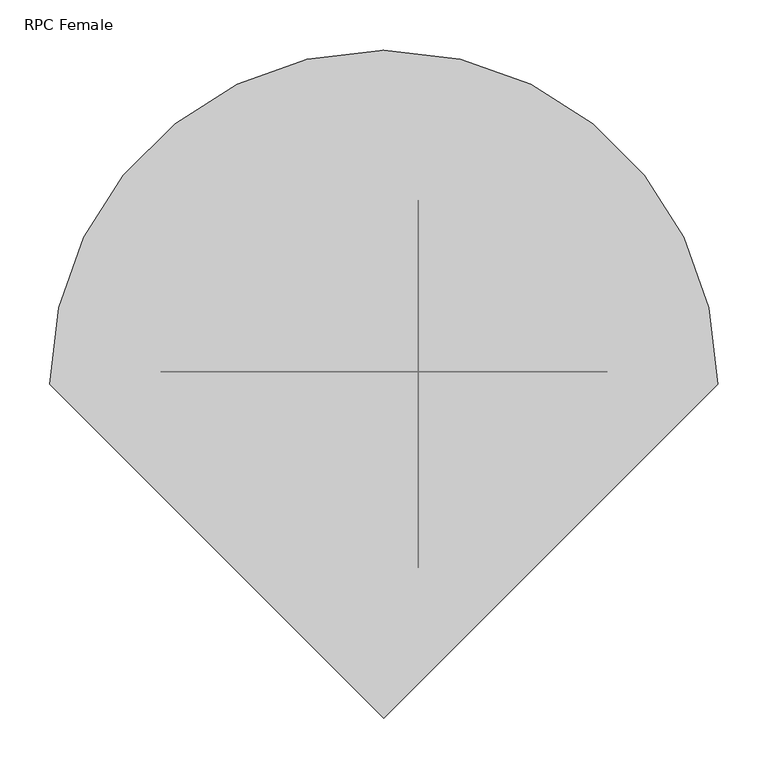
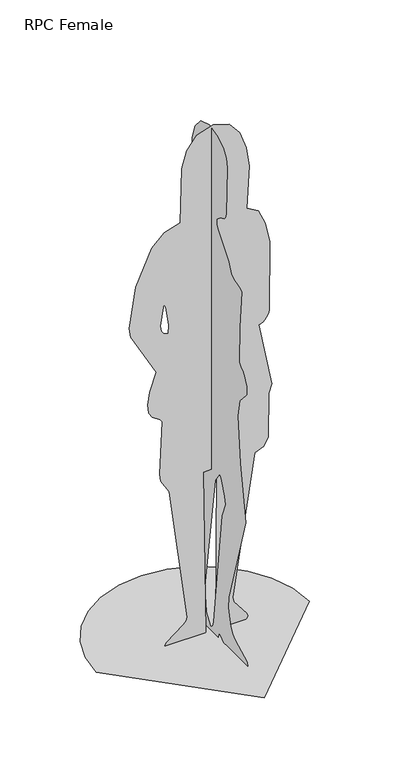
"""IFC4 building model written with IfcOpenShell, lengths in millimetres: proxy geometry, RPC Female : Florence."""

import ifcopenshell
import ifcopenshell.guid

model = None  # the IFC model being written
_history = None  # IfcOwnerHistory: only IFC2X3 demands one
_inside = {}  # id of a spatial element -> (the spatial element, [elements in it])
_under = {}  # id of a project, library or spatial element -> (it, [spatial elements below it])
_declared = {}  # id of a project -> (the project, [libraries it declares])
_typed = {}  # id of a type object -> (the type object, [elements of that type])
_made_of = {}  # id of a material, layer set ... -> (it, [elements and type objects made of it])


def new_model(schema):
    """Start an empty IFC model of exactly this schema.

    Asked for "IFC4X3", IfcOpenShell would pick the latest addendum, in which some entities
    have other attributes; the version numbers below select the first issue.
    IFC2X3 requires an IfcOwnerHistory on every rooted entity: one is made here for all.
    """
    global model, _history
    if schema == "IFC4X3":
        model = ifcopenshell.file(schema_version=(4, 3, 0, 0))
    else:
        model = ifcopenshell.file(schema=schema)
    _inside.clear()
    _under.clear()
    _declared.clear()
    _typed.clear()
    _made_of.clear()
    _history = None
    if model.schema == "IFC2X3":
        org = make("IfcOrganization", Name="unknown")
        user = make(
            "IfcPersonAndOrganization",
            ThePerson=make("IfcPerson", FamilyName="unknown"),
            TheOrganization=org,
        )
        app = make(
            "IfcApplication",
            ApplicationDeveloper=org,
            Version="unknown",
            ApplicationFullName="unknown",
            ApplicationIdentifier="unknown",
        )
        _history = make(
            "IfcOwnerHistory",
            OwningUser=user,
            OwningApplication=app,
            ChangeAction="ADDED",
            CreationDate=0,
        )
    return model


def make(cls, **values):
    """One entity of the class cls with the attributes given. An attribute that is None is left unset."""
    return model.create_entity(
        cls, **{name: value for name, value in values.items() if value is not None}
    )


def rooted(cls, **values):
    """An entity with a GlobalId (a new one), such as an element, a storey or a relation."""
    return make(cls, GlobalId=ifcopenshell.guid.new(), OwnerHistory=_history, **values)


def si_unit(unit_type, name, prefix=None):
    """IfcSIUnit, for example si_unit("LENGTHUNIT", "METRE", prefix="MILLI")."""
    return make("IfcSIUnit", UnitType=unit_type, Prefix=prefix, Name=name)


def assignment(units):
    """IfcUnitAssignment: the units of a project."""
    return None if units is None else make("IfcUnitAssignment", Units=units)


def point(xyz):
    """IfcCartesianPoint."""
    return None if xyz is None else make("IfcCartesianPoint", Coordinates=xyz)


def direction(xyz):
    """IfcDirection."""
    return None if xyz is None else make("IfcDirection", DirectionRatios=xyz)


def frame(location, z_axis=None, x_axis=None):
    """IfcAxis2Placement3D, a coordinate frame: its origin and axes. An axis left out is left unset."""
    return make(
        "IfcAxis2Placement3D",
        Location=point(location),
        Axis=direction(z_axis),
        RefDirection=direction(x_axis),
    )


def origin():
    """The frame at (0, 0, 0) with its axes left unset."""
    return frame((0.0, 0.0, 0.0))


def place(relative_to, where):
    """IfcLocalPlacement: puts the frame where relative to a parent placement (None: the world)."""
    return make(
        "IfcLocalPlacement", PlacementRelTo=relative_to, RelativePlacement=where
    )


def context(
    kind, dimensions, precision=None, world=None, true_north=None, identifier=None
):
    """IfcGeometricRepresentationContext, for example the 3D "Model" context."""
    return make(
        "IfcGeometricRepresentationContext",
        ContextIdentifier=identifier,
        ContextType=kind,
        CoordinateSpaceDimension=dimensions,
        Precision=precision,
        WorldCoordinateSystem=world,
        TrueNorth=true_north,
    )


def project(units=None, contexts=None):
    """IfcProject with its units and contexts."""
    return rooted(
        "IfcProject",
        Name="project",
        RepresentationContexts=contexts,
        UnitsInContext=assignment(units),
    )


def spatial(cls, under=None, at=None, **own):
    """A site, building, storey or space (cls), placed at a placement, below another one or the project."""
    s = rooted(cls, ObjectPlacement=at, **own)
    if under is not None:
        _under.setdefault(under.id(), (under, []))[1].append(s)
    return s


def point_list(points):
    """IfcCartesianPointList2D or 3D."""
    cls = (
        "IfcCartesianPointList2D" if len(points[0]) == 2 else "IfcCartesianPointList3D"
    )
    return make(cls, CoordList=points)


def triangles(points, corners, closed=None, point_numbers=None):
    """IfcTriangulatedFaceSet: each triangle names its three corners, points numbered from 1."""
    return make(
        "IfcTriangulatedFaceSet",
        Coordinates=point_list(points),
        Closed=closed,
        CoordIndex=corners,
        PnIndex=point_numbers,
    )


def shape(context_of_items, identifier, shape_type, items):
    """IfcShapeRepresentation: the items that make up one representation, for example the "Body"."""
    return make(
        "IfcShapeRepresentation",
        ContextOfItems=context_of_items,
        RepresentationIdentifier=identifier,
        RepresentationType=shape_type,
        Items=items,
    )


def source(mapping_origin, context_of_items, identifier, shape_type, items):
    """IfcRepresentationMap: a shape defined once, which mapped items show again and again."""
    return make(
        "IfcRepresentationMap",
        MappingOrigin=mapping_origin,
        MappedRepresentation=shape(context_of_items, identifier, shape_type, items),
    )


def transform(
    local_origin,
    x_axis=None,
    y_axis=None,
    z_axis=None,
    scale=None,
    scale2=None,
    scale3=None,
    uniform=True,
):
    """IfcCartesianTransformationOperator3D, or its non-uniform kind. x_axis, y_axis, z_axis: its Axis1, 2, 3."""
    if uniform:
        return make(
            "IfcCartesianTransformationOperator3D",
            Axis1=direction(x_axis),
            Axis2=direction(y_axis),
            LocalOrigin=point(local_origin),
            Scale=scale,
            Axis3=direction(z_axis),
        )
    return make(
        "IfcCartesianTransformationOperator3DnonUniform",
        Axis1=direction(x_axis),
        Axis2=direction(y_axis),
        LocalOrigin=point(local_origin),
        Scale=scale,
        Axis3=direction(z_axis),
        Scale2=scale2,
        Scale3=scale3,
    )


def mapped(mapping_source, mapping_target):
    """IfcMappedItem: shows the shape of a source again, moved by a transform."""
    return make(
        "IfcMappedItem", MappingSource=mapping_source, MappingTarget=mapping_target
    )


def made_of(thing, what):
    """Note that an element or type object is made of a material, layer set ...; save() writes the relation."""
    if what is not None:
        _made_of.setdefault(what.id(), (what, []))[1].append(thing)
    return thing


def element(
    cls,
    number,
    at=None,
    inside=None,
    cuts=None,
    type_object=None,
    material=None,
    context=None,
    identifier="Body",
    shape_type=None,
    held_by="IfcProductDefinitionShape",
    body=None,
    shapes=None,
    **own,
):
    """One element of the class cls, such as IfcWall. Its Tag is "e" and its number.

    at: its placement. inside: the storey or other place that contains it. cuts: it is an
    opening in that element (IfcRelVoidsElement). A single representation is given by context,
    identifier, shape_type and body (its items); several are given by shapes. held_by: the class
    of the entity that holds the representations. save() writes the other relations.
    """
    e = rooted(cls, Tag="e%d" % number, ObjectPlacement=at, **own)
    if body is not None:
        shapes = [shape(context, identifier, shape_type, body)]
    if shapes is not None:
        e.Representation = make(held_by, Representations=shapes)
    if inside is not None:
        _inside.setdefault(inside.id(), (inside, []))[1].append(e)
    if cuts is not None:
        rooted(
            "IfcRelVoidsElement", RelatingBuildingElement=cuts, RelatedOpeningElement=e
        )
    if type_object is not None:
        _typed.setdefault(type_object.id(), (type_object, []))[1].append(e)
    return made_of(e, material)


def aggregate(whole, parts):
    """IfcRelAggregates: a whole, such as a stair, and the parts it consists of."""
    return rooted("IfcRelAggregates", RelatingObject=whole, RelatedObjects=parts)


def save(model, path):
    """Write the relations noted so far, then the file.

    IfcRelAggregates (storeys below a building ...), IfcRelContainedInSpatialStructure (elements
    in a storey), IfcRelDefinesByType, IfcRelAssociatesMaterial and IfcRelDeclares: one each for
    every whole, place, type object, material and project.
    """
    for whole, parts in _under.values():
        aggregate(whole, parts)
    for where, things in _inside.values():
        rooted(
            "IfcRelContainedInSpatialStructure",
            RelatedElements=things,
            RelatingStructure=where,
        )
    for kind, things in _typed.values():
        rooted("IfcRelDefinesByType", RelatedObjects=things, RelatingType=kind)
    for what, things in _made_of.values():
        rooted("IfcRelAssociatesMaterial", RelatedObjects=things, RelatingMaterial=what)
    for by, libraries in _declared.values():
        rooted("IfcRelDeclares", RelatingContext=by, RelatedDefinitions=libraries)
    model.write(path)


def rpc_female_692637f3(model_context):
    return source(origin(), model_context, "Body", "Tessellation", [
        triangles([(334.1038436, 0.0002006, 4.67e-05), (325.2712069, 76.554684, 4.67e-05), (300.1160563, 146.8577329, 4.67e-05), (260.6525312, 208.8950799, 4.67e-05), (208.8950436, 260.6526402, 4.67e-05), (146.8576239, 300.1161108, 4.67e-05), (76.5545841, 325.2713159, 4.67e-05), (0.0001119, 334.1039526, 4.67e-05), (-76.5543661, 325.2713159, 4.67e-05), (-146.8574241, 300.1161471, 4.67e-05), (-208.8947893, 260.6526402, 4.67e-05), (-260.6523677, 208.8951526, 4.67e-05), (-300.1157837, 146.8577238, 4.67e-05), (-325.2709888, 76.5546749, 4.67e-05), (-334.1036256, 0.0002063, 4.67e-05), (0.0001354, -334.1035166, 4.67e-05), (34.5735982, -6.9369908, 510.5862036), (34.5736005, 50.0894208, 122.5869578), (34.5736005, 40.8608144, 46.3929486), (34.5735982, 17.1569787, 11.3406073), (34.5735982, 7.4077424, 20.0668393), (34.5735982, 1.2816647, 37.4286861), (34.5735982, -2.1837537, 60.406083), (34.573596, -46.4921976, 417.5145226), (34.573596, -63.110333, 464.5403223), (34.573596, -60.1161389, 490.2851171), (34.573596, -39.0453865, 536.4626401), (34.573596, -31.9759211, 546.3433597), (34.5736051, 133.6635619, 4.67e-05), (34.5736051, 131.2497012, 427.6552917), (34.5736028, 105.4428553, 516.402818), (34.5736051, 133.6330768, 904.8776161), (34.5736051, 118.5363239, 971.9484495), (34.5736051, 119.0610557, 980.9675211), (34.5736051, 126.7253499, 988.4865389), (34.5736073, 167.3251791, 1010.3459604), (34.5736073, 178.3172225, 1020.1671633), (34.5736073, 183.8335464, 1032.6394398), (34.5736073, 170.1064229, 1269.4988194), (34.5736073, 153.1875791, 1316.4971134), (34.5736051, 126.3412163, 1357.63312), (34.5736051, 116.7179574, 1573.3395756), (34.5736028, 100.9948892, 1620.5182365), (34.5736028, 71.8814228, 1654.7582977), (34.5736005, 25.3458139, 1670.9407402), (34.573596, -21.8028775, 1659.2649994), (34.573596, -51.3715418, 1640.0022217), (34.5735937, -67.2787558, 1615.437006), (34.5735937, -73.4430507, 1587.8543873), (34.5735937, -67.1164838, 1429.4550442), (34.573596, -62.6125163, 1414.6470818), (34.573596, -56.0058929, 1408.6359661), (34.573596, -33.6371819, 1398.6160835), (34.5735982, -16.4512737, 1382.4130028), (34.5735982, -16.5742143, 1366.5170254), (34.573596, -23.8041702, 1350.9894848), (34.5735937, -80.3271009, 1279.6723263), (34.5735937, -93.6682833, 1248.0555061), (34.5735937, -101.8993307, 1241.9481754), (34.5735914, -113.2375739, 1237.3922035), (34.5735914, -125.7355211, 1233.7834122), (34.5735914, -137.445871, 1230.5184952), (34.5735914, -146.4210681, 1226.9929836), (34.5735914, -150.7137475, 1222.6031353), (34.5735914, -148.5625071, 1190.0747429), (34.5735914, -140.3131288, 1099.0845119), (34.5735914, -138.7464003, 982.8324509), (34.5735914, -146.619339, 972.1617359), (34.5735892, -156.6982296, 965.1524254), (34.5735892, -165.5360078, 953.6295095), (34.5735892, -177.5233393, 924.4368147), (34.5735892, -179.6904672, 910.463249), (34.5735892, -178.6515408, 899.3693041), (34.5735892, -173.9153837, 893.0032682), (34.5735914, -141.1932077, 856.8173229), (34.5735914, -128.9730324, 798.8474602), (34.5735914, -142.8069082, 650.4621861), (34.5735892, -172.1239596, 470.1701385), (34.5735937, -80.165383, 167.8524907), (34.5735937, -77.6113328, 131.7844796), (34.5735937, -91.6647991, 75.8743931), (34.5735937, -102.4531668, 58.8461219), (34.5735914, -116.401843, 46.2735109), (34.5735892, -182.1041825, 14.070202), (34.5735892, -183.8332739, 4.67e-05), (34.573596, -53.8341595, 4.67e-05), (34.573596, -35.7947333, 12.7326758), (34.573596, -29.2463276, 15.4350465), (34.573596, -27.5084158, 14.8404334), (34.573596, -26.3930815, 13.6010264), (34.573596, -23.0174154, 4.67e-05), (-109.094313, 12.6252593, 1123.2807821), (-99.0692164, 12.6252548, 1062.4456146), (-101.4218071, 12.6252536, 1032.213085), (-115.6875607, 12.6252536, 1036.9381599), (-123.3610839, 12.6252559, 1049.3745375), (-125.9345188, 12.6252559, 1066.9140919), (-115.0698113, 12.6252593, 1135.9380037), (142.5673516, 12.6251787, 0.0), (147.4016405, 12.6251787, 9.7557227), (144.3531438, 12.6251798, 20.3925416), (104.8323548, 12.6251855, 72.3575519), (100.9956885, 12.6251855, 87.8546938), (169.3636811, 12.6252093, 543.0591125), (197.666532, 12.6252093, 555.605367), (211.7994085, 12.6252093, 579.9655443), (214.3379708, 12.6252173, 724.0128565), (223.4012803, 12.6252196, 753.7932335), (181.7748058, 12.6252343, 962.6080313), (189.3709628, 12.6252332, 963.9546787), (195.9600047, 12.6252332, 967.6156471), (201.5896029, 12.6252343, 973.0224392), (206.3074654, 12.6252343, 979.6063396), (210.1614997, 12.6252332, 986.7992872), (213.1992504, 12.6252332, 994.0323486), (215.4685159, 12.6252343, 1000.7370993), (216.7847147, 12.6252479, 1226.3016014), (203.5876096, 12.6252536, 1292.6408661), (180.5930284, 12.625257, 1341.5987789), (145.6075276, 12.6252582, 1362.4953232), (152.3856295, 12.6252672, 1500.6374725), (142.6607235, 12.6252718, 1563.7968441), (122.5370971, 12.6252763, 1620.2490669), (89.370735, 12.625282, 1660.8358337), (40.5176895, 12.6252843, 1676.4), (-11.7228571, 12.6252854, 1659.2202347), (-43.4643846, 12.6252854, 1619.483416), (-59.5217757, 12.6252831, 1565.8930824), (-63.2073292, 12.6252718, 1387.0617016), (-114.1079968, 12.6252741, 1371.9761398), (-153.4323498, 12.6252729, 1333.9056438), (-202.7226188, 12.6252695, 1222.3996593), (-223.4010259, 12.6252627, 1092.6907888), (-219.1643114, 12.6252604, 1062.1448336), (-139.8068642, 12.6252468, 917.9959288), (-160.1374456, 12.6252457, 858.7674219), (-166.230642, 12.6252434, 817.4798985), (-162.0168367, 12.6252411, 790.3472523), (-151.4263857, 12.6252389, 773.5839586), (-126.837407, 12.6252377, 756.0219492), (-120.6996275, 12.6252366, 747.6516026), (-128.6616143, 12.6252264, 575.4503403), (-125.4420706, 12.6252252, 551.8412436), (-98.6846832, 12.6252218, 508.0167383), (-41.8822682, 12.6251934, 71.4770234), (-45.3585504, 12.6251912, 61.0228059), (-53.9451629, 12.6251912, 51.2209333), (-105.6091242, 12.6251923, 11.6815362), (-114.4080966, 12.6251923, 0.0), (16.5202489, 12.6251855, 0.0), (7.7624049, 12.6252184, 535.4248037), (51.4361137, 12.6252162, 536.7896187), (47.7042875, 12.6251844, 0.0)], [[15, 16, 1], [14, 15, 1], [14, 1, 2], [13, 14, 2], [13, 2, 3], [13, 3, 4], [12, 13, 4], [11, 12, 4], [11, 4, 5], [11, 5, 6], [11, 6, 7], [11, 7, 8], [11, 8, 9], [11, 9, 10], [91, 29, 20], [91, 20, 21], [19, 20, 29], [84, 85, 86], [83, 84, 86], [82, 83, 86], [91, 21, 22], [90, 91, 22], [18, 19, 29], [18, 29, 30], [18, 30, 31], [17, 18, 31], [89, 90, 22], [28, 17, 31], [81, 82, 86], [81, 86, 87], [81, 87, 88], [89, 22, 23], [88, 89, 23], [81, 88, 23], [80, 81, 23], [79, 80, 23], [79, 23, 24], [79, 24, 25], [78, 79, 25], [78, 25, 26], [78, 26, 27], [77, 78, 27], [77, 27, 28], [77, 28, 31], [76, 77, 31], [76, 31, 32], [75, 76, 32], [75, 32, 33], [74, 75, 33], [74, 33, 34], [73, 74, 34], [72, 73, 34], [71, 72, 34], [70, 71, 34], [69, 70, 34], [68, 69, 34], [67, 68, 34], [66, 67, 34], [66, 34, 35], [65, 66, 35], [65, 35, 36], [65, 36, 37], [65, 37, 38], [65, 38, 39], [64, 65, 39], [63, 64, 39], [62, 63, 39], [61, 62, 39], [60, 61, 39], [59, 60, 39], [58, 59, 39], [57, 58, 39], [57, 39, 40], [57, 40, 41], [56, 57, 41], [55, 56, 41], [54, 55, 41], [53, 54, 41], [53, 41, 42], [52, 53, 42], [51, 52, 42], [50, 51, 42], [50, 42, 43], [50, 43, 44], [50, 44, 45], [50, 45, 46], [49, 50, 46], [49, 46, 47], [49, 47, 48], [148, 149, 150], [147, 148, 150], [146, 147, 150], [145, 146, 150], [145, 150, 151], [144, 145, 151], [94, 104, 105], [94, 105, 106], [94, 106, 107], [94, 107, 108], [94, 108, 109], [93, 94, 109], [153, 99, 100], [153, 100, 101], [153, 101, 102], [143, 144, 151], [142, 143, 151], [153, 102, 103], [152, 153, 103], [152, 103, 104], [152, 104, 94], [151, 152, 94], [151, 94, 95], [92, 93, 109], [92, 109, 110], [92, 110, 111], [92, 111, 112], [92, 112, 113], [92, 113, 114], [92, 114, 115], [92, 115, 116], [92, 116, 117], [92, 117, 118], [98, 92, 118], [98, 118, 119], [98, 119, 120], [98, 120, 121], [98, 121, 122], [98, 122, 123], [98, 123, 124], [98, 124, 125], [141, 142, 151], [141, 151, 95], [140, 141, 95], [139, 140, 95], [138, 139, 95], [125, 126, 127], [125, 127, 128], [129, 130, 131], [129, 131, 132], [129, 132, 133], [129, 133, 134], [136, 137, 138], [135, 136, 138], [135, 138, 95], [134, 135, 95], [134, 95, 96], [134, 96, 97], [125, 128, 129], [98, 125, 129], [98, 129, 134], [98, 134, 97]], closed=False),
    ])


if __name__ == "__main__":
    model = new_model("IFC4")
    model_context = context("Model", 3, world=origin())
    ifc_project = project(units=[si_unit("LENGTHUNIT", "METRE", prefix="MILLI")], contexts=[model_context])
    site = spatial("IfcSite", under=ifc_project)
    building = spatial("IfcBuilding", under=site)
    placement = place(None, origin())
    rpc_female_shape = rpc_female_692637f3(model_context)
    element("IfcBuildingElementProxy", 1, Name="RPC Female : Florence", ObjectType="RPC Female : Florence", at=placement, inside=building, context=model_context, shape_type="MappedRepresentation", body=[
        mapped(rpc_female_shape, transform((0.0, 0.0, 0.0), x_axis=(1.0, 0.0, 0.0), y_axis=(0.0, 1.0, 0.0), z_axis=(0.0, 0.0, 1.0))),
    ])
    save(model, "model.ifc")

# Revit data of these elements
# Type "RPC Female : Florence"
#   built-in parameter 1005198 = "{2, 15},{22, RPC-8-G3AF-G2XX-UFB5-G},{1, 0},{1, 0},{2, 15},{1, 8},{5, Color},{1, 0},{1, 0},{3, 0.8},{3, 0.8},{3, 0.8},{1, 8},{7, BBoxMin},{1, 0},{1, 0},{1, 0},{1, 0},{1, 0},{1, 8},{7, BBoxMax},{1, 0},{1, 0},{1, 0},{1, 0},{1, 0},{2, 11},{9, RPCTypeId},{1, 0},{1, 0},{22, RPC-8-G3AF-G2XX-UFB5-G},{1, 6},{14, RPCPlantHeight},{1, 0},{1, 0},{3, 5.5},{2, 11},{7, keyword},{1, 0},{1, 0},{42, :RPCs:People [Business-Asian]:Geometry:RPC},{2, 11},{8, category},{1, 0},{1, 0},{23, People [Business-Asian]},{2, 11},{12, LocalizedUID},{1, 0},{1, 0},{8, Florence},{2, 14},{6, Height},{1, 0},{1, 0},{3, 5.5},{1, 2},{16, Cast Reflections},{1, 0},{1, 0},{1, 0},{1, 2},{6, Jitter},{1, 0},{1, 0},{1, 1},{1, 2},{9, Billboard},{1, 0},{1, 0},{1, 0},{1, 2},{12, Cast Shadows},{1, 0},{1, 0},{1, 1},{1, 2},{20, Apply Filter Effects},{1, 0},{1, 0},{1, 0},{2, 11},{28, Apply Filter Effects-Text-FC},{1, 0},{1, 0},{4, None},{21, assetlibrary_base.fbx},{1, 5},"
#   built-in parameter 1005195 = "RPC-8-G3AF-G2XX-UFB5-G"
#   Height = 0
